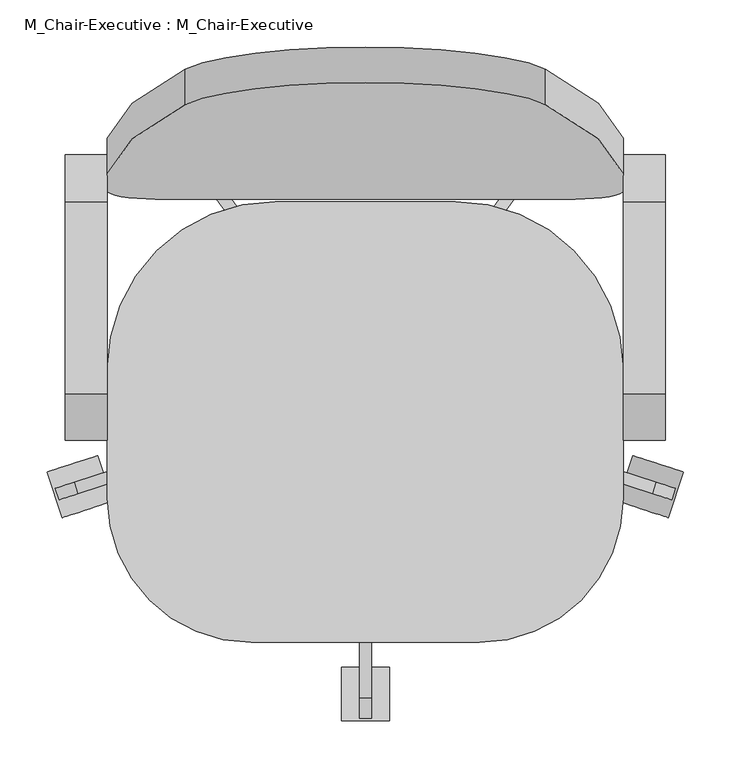
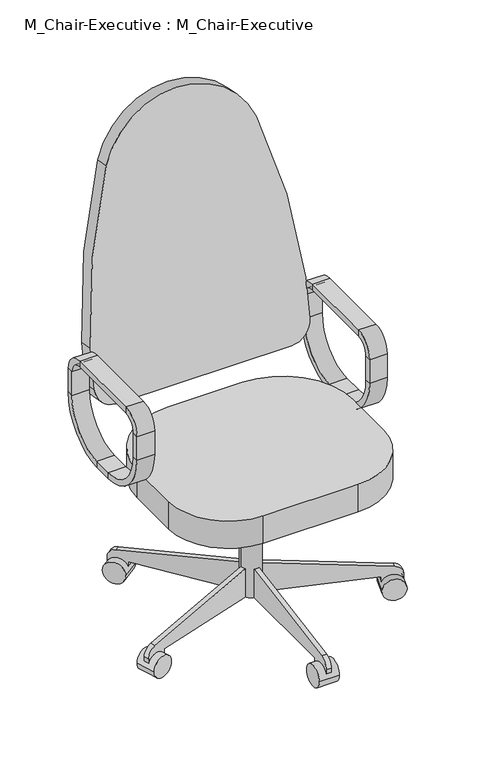
"""IFC4 building model written with IfcOpenShell, lengths in millimetres: furniture geometry, M_Chair-Executive : M_Chair-Executive."""

import ifcopenshell
import ifcopenshell.guid

model = None  # the IFC model being written
_history = None  # IfcOwnerHistory: only IFC2X3 demands one
_inside = {}  # id of a spatial element -> (the spatial element, [elements in it])
_under = {}  # id of a project, library or spatial element -> (it, [spatial elements below it])
_declared = {}  # id of a project -> (the project, [libraries it declares])
_typed = {}  # id of a type object -> (the type object, [elements of that type])
_made_of = {}  # id of a material, layer set ... -> (it, [elements and type objects made of it])


def new_model(schema):
    """Start an empty IFC model of exactly this schema.

    Asked for "IFC4X3", IfcOpenShell would pick the latest addendum, in which some entities
    have other attributes; the version numbers below select the first issue.
    IFC2X3 requires an IfcOwnerHistory on every rooted entity: one is made here for all.
    """
    global model, _history
    if schema == "IFC4X3":
        model = ifcopenshell.file(schema_version=(4, 3, 0, 0))
    else:
        model = ifcopenshell.file(schema=schema)
    _inside.clear()
    _under.clear()
    _declared.clear()
    _typed.clear()
    _made_of.clear()
    _history = None
    if model.schema == "IFC2X3":
        org = make("IfcOrganization", Name="unknown")
        user = make(
            "IfcPersonAndOrganization",
            ThePerson=make("IfcPerson", FamilyName="unknown"),
            TheOrganization=org,
        )
        app = make(
            "IfcApplication",
            ApplicationDeveloper=org,
            Version="unknown",
            ApplicationFullName="unknown",
            ApplicationIdentifier="unknown",
        )
        _history = make(
            "IfcOwnerHistory",
            OwningUser=user,
            OwningApplication=app,
            ChangeAction="ADDED",
            CreationDate=0,
        )
    return model


def make(cls, **values):
    """One entity of the class cls with the attributes given. An attribute that is None is left unset."""
    return model.create_entity(
        cls, **{name: value for name, value in values.items() if value is not None}
    )


def rooted(cls, **values):
    """An entity with a GlobalId (a new one), such as an element, a storey or a relation."""
    return make(cls, GlobalId=ifcopenshell.guid.new(), OwnerHistory=_history, **values)


def si_unit(unit_type, name, prefix=None):
    """IfcSIUnit, for example si_unit("LENGTHUNIT", "METRE", prefix="MILLI")."""
    return make("IfcSIUnit", UnitType=unit_type, Prefix=prefix, Name=name)


def assignment(units):
    """IfcUnitAssignment: the units of a project."""
    return None if units is None else make("IfcUnitAssignment", Units=units)


def point(xyz):
    """IfcCartesianPoint."""
    return None if xyz is None else make("IfcCartesianPoint", Coordinates=xyz)


def direction(xyz):
    """IfcDirection."""
    return None if xyz is None else make("IfcDirection", DirectionRatios=xyz)


def frame(location, z_axis=None, x_axis=None):
    """IfcAxis2Placement3D, a coordinate frame: its origin and axes. An axis left out is left unset."""
    return make(
        "IfcAxis2Placement3D",
        Location=point(location),
        Axis=direction(z_axis),
        RefDirection=direction(x_axis),
    )


def frame_2d(location, x_axis=None):
    """IfcAxis2Placement2D, a coordinate frame in the plane: its origin and x axis."""
    return make(
        "IfcAxis2Placement2D", Location=point(location), RefDirection=direction(x_axis)
    )


def origin():
    """The frame at (0, 0, 0) with its axes left unset."""
    return frame((0.0, 0.0, 0.0))


def place(relative_to, where):
    """IfcLocalPlacement: puts the frame where relative to a parent placement (None: the world)."""
    return make(
        "IfcLocalPlacement", PlacementRelTo=relative_to, RelativePlacement=where
    )


def context(
    kind, dimensions, precision=None, world=None, true_north=None, identifier=None
):
    """IfcGeometricRepresentationContext, for example the 3D "Model" context."""
    return make(
        "IfcGeometricRepresentationContext",
        ContextIdentifier=identifier,
        ContextType=kind,
        CoordinateSpaceDimension=dimensions,
        Precision=precision,
        WorldCoordinateSystem=world,
        TrueNorth=true_north,
    )


def project(units=None, contexts=None):
    """IfcProject with its units and contexts."""
    return rooted(
        "IfcProject",
        Name="project",
        RepresentationContexts=contexts,
        UnitsInContext=assignment(units),
    )


def spatial(cls, under=None, at=None, **own):
    """A site, building, storey or space (cls), placed at a placement, below another one or the project."""
    s = rooted(cls, ObjectPlacement=at, **own)
    if under is not None:
        _under.setdefault(under.id(), (under, []))[1].append(s)
    return s


def polyline(points):
    """IfcPolyline through the points."""
    return make("IfcPolyline", Points=[point(p) for p in points])


def circle_curve(where, radius):
    """IfcCircle in the frame where."""
    return make("IfcCircle", Position=where, Radius=radius)


def trimmed(basis, trim1, trim2, sense, master):
    """IfcTrimmedCurve: the piece of a basis curve between two trims."""
    return make(
        "IfcTrimmedCurve",
        BasisCurve=basis,
        Trim1=trim1,
        Trim2=trim2,
        SenseAgreement=sense,
        MasterRepresentation=master,
    )


def segment(curve, same_sense, transition):
    """IfcCompositeCurveSegment."""
    return make(
        "IfcCompositeCurveSegment",
        Transition=transition,
        SameSense=same_sense,
        ParentCurve=curve,
    )


def composite_curve(segments, self_intersect=None):
    """IfcCompositeCurve: segments joined end to end."""
    return make("IfcCompositeCurve", Segments=segments, SelfIntersect=self_intersect)


def outline(outer, holes=None, kind="AREA"):
    """IfcArbitraryClosedProfileDef: a profile drawn as a closed curve; with holes, ...WithVoids."""
    if holes is None:
        return make("IfcArbitraryClosedProfileDef", ProfileType=kind, OuterCurve=outer)
    return make(
        "IfcArbitraryProfileDefWithVoids",
        ProfileType=kind,
        OuterCurve=outer,
        InnerCurves=holes,
    )


def extrude(swept, where, along, depth):
    """IfcExtrudedAreaSolid: the profile swept, set in the frame where, extruded along a direction by depth."""
    return make(
        "IfcExtrudedAreaSolid",
        SweptArea=swept,
        Position=where,
        ExtrudedDirection=direction(along),
        Depth=depth,
    )


def shape(context_of_items, identifier, shape_type, items):
    """IfcShapeRepresentation: the items that make up one representation, for example the "Body"."""
    return make(
        "IfcShapeRepresentation",
        ContextOfItems=context_of_items,
        RepresentationIdentifier=identifier,
        RepresentationType=shape_type,
        Items=items,
    )


def source(mapping_origin, context_of_items, identifier, shape_type, items):
    """IfcRepresentationMap: a shape defined once, which mapped items show again and again."""
    return make(
        "IfcRepresentationMap",
        MappingOrigin=mapping_origin,
        MappedRepresentation=shape(context_of_items, identifier, shape_type, items),
    )


def transform(
    local_origin,
    x_axis=None,
    y_axis=None,
    z_axis=None,
    scale=None,
    scale2=None,
    scale3=None,
    uniform=True,
):
    """IfcCartesianTransformationOperator3D, or its non-uniform kind. x_axis, y_axis, z_axis: its Axis1, 2, 3."""
    if uniform:
        return make(
            "IfcCartesianTransformationOperator3D",
            Axis1=direction(x_axis),
            Axis2=direction(y_axis),
            LocalOrigin=point(local_origin),
            Scale=scale,
            Axis3=direction(z_axis),
        )
    return make(
        "IfcCartesianTransformationOperator3DnonUniform",
        Axis1=direction(x_axis),
        Axis2=direction(y_axis),
        LocalOrigin=point(local_origin),
        Scale=scale,
        Axis3=direction(z_axis),
        Scale2=scale2,
        Scale3=scale3,
    )


def mapped(mapping_source, mapping_target):
    """IfcMappedItem: shows the shape of a source again, moved by a transform."""
    return make(
        "IfcMappedItem", MappingSource=mapping_source, MappingTarget=mapping_target
    )


def made_of(thing, what):
    """Note that an element or type object is made of a material, layer set ...; save() writes the relation."""
    if what is not None:
        _made_of.setdefault(what.id(), (what, []))[1].append(thing)
    return thing


def element(
    cls,
    number,
    at=None,
    inside=None,
    cuts=None,
    type_object=None,
    material=None,
    context=None,
    identifier="Body",
    shape_type=None,
    held_by="IfcProductDefinitionShape",
    body=None,
    shapes=None,
    **own,
):
    """One element of the class cls, such as IfcWall. Its Tag is "e" and its number.

    at: its placement. inside: the storey or other place that contains it. cuts: it is an
    opening in that element (IfcRelVoidsElement). A single representation is given by context,
    identifier, shape_type and body (its items); several are given by shapes. held_by: the class
    of the entity that holds the representations. save() writes the other relations.
    """
    e = rooted(cls, Tag="e%d" % number, ObjectPlacement=at, **own)
    if body is not None:
        shapes = [shape(context, identifier, shape_type, body)]
    if shapes is not None:
        e.Representation = make(held_by, Representations=shapes)
    if inside is not None:
        _inside.setdefault(inside.id(), (inside, []))[1].append(e)
    if cuts is not None:
        rooted(
            "IfcRelVoidsElement", RelatingBuildingElement=cuts, RelatedOpeningElement=e
        )
    if type_object is not None:
        _typed.setdefault(type_object.id(), (type_object, []))[1].append(e)
    return made_of(e, material)


def aggregate(whole, parts):
    """IfcRelAggregates: a whole, such as a stair, and the parts it consists of."""
    return rooted("IfcRelAggregates", RelatingObject=whole, RelatedObjects=parts)


def save(model, path):
    """Write the relations noted so far, then the file.

    IfcRelAggregates (storeys below a building ...), IfcRelContainedInSpatialStructure (elements
    in a storey), IfcRelDefinesByType, IfcRelAssociatesMaterial and IfcRelDeclares: one each for
    every whole, place, type object, material and project.
    """
    for whole, parts in _under.values():
        aggregate(whole, parts)
    for where, things in _inside.values():
        rooted(
            "IfcRelContainedInSpatialStructure",
            RelatedElements=things,
            RelatingStructure=where,
        )
    for kind, things in _typed.values():
        rooted("IfcRelDefinesByType", RelatedObjects=things, RelatingType=kind)
    for what, things in _made_of.values():
        rooted("IfcRelAssociatesMaterial", RelatedObjects=things, RelatingMaterial=what)
    for by, libraries in _declared.values():
        rooted("IfcRelDeclares", RelatingContext=by, RelatedDefinitions=libraries)
    model.write(path)


def plane_surface(at):
    """IfcPlane: the flat surface through the origin of the frame at, square to its z axis."""
    return make("IfcPlane", Position=at)


def cylinder_surface(at, radius):
    """IfcCylindricalSurface: all points at the distance radius from the z axis of the frame at."""
    return make("IfcCylindricalSurface", Position=at, Radius=radius)


def revolved_surface(curve, axis_point, axis_direction):
    """IfcSurfaceOfRevolution: the curve turned about the line through axis_point along axis_direction."""
    return make(
        "IfcSurfaceOfRevolution",
        SweptCurve=make("IfcArbitraryOpenProfileDef", ProfileType="CURVE", Curve=curve),
        AxisPosition=make("IfcAxis1Placement", Location=point(axis_point), Axis=direction(axis_direction)),
    )


def advanced_brep(points, edges, surfaces, faces):
    """IfcAdvancedBrep: a solid bounded by faces that lie on surfaces and meet in shared edges.

    An edge is (start, end): straight between two places in points (the first is 0);
    or (start, end, curve); or (start, end, curve, False) where it runs against its curve.
    A face is (place in surfaces, loops), or (place, loops, False) where it looks against
    its surface's normal. A loop lists edges by number (the first is 1), with a minus sign
    where the edge is run from its end to its start. The first loop is the outer one.
    """
    corners = [point(p) for p in points]
    vertices = [make("IfcVertexPoint", VertexGeometry=c) for c in corners]
    made = []
    for start, end, *more in edges:
        made.append(
            make(
                "IfcEdgeCurve",
                EdgeStart=vertices[start],
                EdgeEnd=vertices[end],
                EdgeGeometry=more[0] if more else make("IfcPolyline", Points=[corners[start], corners[end]]),
                SameSense=more[1] if len(more) > 1 else True,
            )
        )
    hull = []
    for where, loops, *sense in faces:
        bounds = []
        for j, loop in enumerate(loops):
            ring = [make("IfcOrientedEdge", EdgeElement=made[abs(k) - 1], Orientation=k > 0) for k in loop]
            bounds.append(
                make(
                    "IfcFaceOuterBound" if j == 0 else "IfcFaceBound",
                    Bound=make("IfcEdgeLoop", EdgeList=ring),
                    Orientation=True,
                )
            )
        hull.append(make("IfcAdvancedFace", Bounds=bounds, FaceSurface=surfaces[where], SameSense=sense[0] if sense else True))
    return make("IfcAdvancedBrep", Outer=make("IfcClosedShell", CfsFaces=hull))


def m_chair_executive_m_chair_executive_a5be4872(model_context):
    return source(origin(), model_context, "Body", "SolidModel", [
        advanced_brep(
        [(-176.5091803, 217.7873012, 546.1), (-176.5091803, 233.6623012, 546.1), (-176.5091803, 108.0540984, 420.4917972), (-176.5091803, 108.0540984, 436.3667972), (-132.0591803, 217.7873012, 546.1), (-132.0591803, 108.0540984, 436.3667972), (-132.0591803, 233.6623012, 546.1), (-132.0591803, 108.0540984, 420.4917972), (-176.5091803, 217.7873012, 609.6), (-176.5091803, 233.6623012, 609.6), (-132.0591803, 217.7873012, 609.6), (-132.0591803, 233.6623012, 609.6), (-176.5091803, 184.2540984, 643.1332028), (-176.5091803, 184.2540984, 659.0082028), (-132.0591803, 184.2540984, 643.1332028), (-132.0591803, 184.2540984, 659.0082028), (-176.5091803, -18.9459016, 643.1332028), (-176.5091803, -18.9459016, 659.0082028), (-132.0591803, -18.9459016, 643.1332028), (-132.0591803, -18.9459016, 659.0082028), (-176.5091803, -52.4791044, 609.6), (-176.5091803, -68.3541044, 609.6), (-132.0591803, -52.4791044, 609.6), (-132.0591803, -68.3541044, 609.6), (-176.5091803, -52.4791044, 546.1), (-176.5091803, -68.3541044, 546.1), (-132.0591803, -52.4791044, 546.1), (-132.0591803, -68.3541044, 546.1), (-176.5091803, 57.2540984, 436.3667972), (-176.5091803, 57.2540984, 420.4917972), (-132.0591803, 57.2540984, 436.3667972), (-132.0591803, 57.2540984, 420.4917972)],
        [
            (0, 1),
            (1, 2, circle_curve(frame((-176.5091803, 108.0540984, 546.1), z_axis=(-1.0, 0.0, 0.0), x_axis=(0.0, 0.0, -1.0)), 125.6082028)),
            (2, 3),
            (3, 0, circle_curve(frame((-176.5091803, 108.0540984, 546.1), z_axis=(1.0, 0.0, 0.0), x_axis=(0.0, 0.0, -1.0)), 109.7332028)),
            (4, 0),
            (3, 5),
            (5, 4, circle_curve(frame((-132.0591803, 108.0540984, 546.1), z_axis=(1.0, 0.0, 0.0), x_axis=(0.0, 0.0, -1.0)), 109.7332028)),
            (6, 4),
            (5, 7),
            (7, 6, circle_curve(frame((-132.0591803, 108.0540984, 546.1), z_axis=(1.0, 0.0, 0.0), x_axis=(0.0, 0.0, -1.0)), 125.6082028)),
            (1, 6),
            (7, 2),
            (0, 8),
            (8, 9),
            (9, 1),
            (4, 10),
            (10, 8),
            (6, 11),
            (11, 10),
            (9, 11),
            (12, 13),
            (13, 9, circle_curve(frame((-176.5091803, 184.2540984, 609.6), z_axis=(-1.0, 0.0, 0.0), x_axis=(0.0, 1.0, 0.0)), 49.4082028)),
            (8, 12, circle_curve(frame((-176.5091803, 184.2540984, 609.6), z_axis=(1.0, 0.0, 0.0), x_axis=(0.0, 1.0, 0.0)), 33.5332028)),
            (14, 12),
            (10, 14, circle_curve(frame((-132.0591803, 184.2540984, 609.6), z_axis=(1.0, 0.0, 0.0), x_axis=(0.0, 1.0, 0.0)), 33.5332028)),
            (15, 14),
            (11, 15, circle_curve(frame((-132.0591803, 184.2540984, 609.6), z_axis=(1.0, 0.0, 0.0), x_axis=(0.0, 1.0, 0.0)), 49.4082028)),
            (13, 15),
            (12, 16),
            (16, 17),
            (17, 13),
            (14, 18),
            (18, 16),
            (15, 19),
            (19, 18),
            (17, 19),
            (20, 21),
            (21, 17, circle_curve(frame((-176.5091803, -18.9459016, 609.6), z_axis=(-1.0, 0.0, 0.0), x_axis=(0.0, 0.0, 1.0)), 49.4082028)),
            (16, 20, circle_curve(frame((-176.5091803, -18.9459016, 609.6), z_axis=(1.0, 0.0, 0.0), x_axis=(0.0, 0.0, 1.0)), 33.5332028)),
            (22, 20),
            (18, 22, circle_curve(frame((-132.0591803, -18.9459016, 609.6), z_axis=(1.0, 0.0, 0.0), x_axis=(0.0, 0.0, 1.0)), 33.5332028)),
            (23, 22),
            (19, 23, circle_curve(frame((-132.0591803, -18.9459016, 609.6), z_axis=(1.0, 0.0, 0.0), x_axis=(0.0, 0.0, 1.0)), 49.4082028)),
            (21, 23),
            (20, 24),
            (24, 25),
            (25, 21),
            (22, 26),
            (26, 24),
            (23, 27),
            (27, 26),
            (25, 27),
            (28, 29),
            (29, 25, circle_curve(frame((-176.5091803, 57.2540984, 546.1), z_axis=(-1.0, 0.0, 0.0), x_axis=(0.0, -1.0, 0.0)), 125.6082028)),
            (24, 28, circle_curve(frame((-176.5091803, 57.2540984, 546.1), z_axis=(1.0, 0.0, 0.0), x_axis=(0.0, -1.0, 0.0)), 109.7332028)),
            (30, 28),
            (26, 30, circle_curve(frame((-132.0591803, 57.2540984, 546.1), z_axis=(1.0, 0.0, 0.0), x_axis=(0.0, -1.0, 0.0)), 109.7332028)),
            (31, 30),
            (27, 31, circle_curve(frame((-132.0591803, 57.2540984, 546.1), z_axis=(1.0, 0.0, 0.0), x_axis=(0.0, -1.0, 0.0)), 125.6082028)),
            (29, 31),
            (28, 3),
            (2, 29),
            (30, 5),
            (31, 7),
        ],
        [
            plane_surface(frame((-176.5091803, 108.0540984, 546.1), z_axis=(-1.0, 0.0, 0.0), x_axis=(0.0, 0.0, -1.0))),
            revolved_surface(polyline([(-176.5091803, 108.0540984, 436.3667972), (-132.0591803, 108.0540984, 436.3667972)]), (-132.0591803, 108.0540984, 546.1), (-1.0, 0.0, 0.0)),
            plane_surface(frame((-132.0591803, 108.0540984, 546.1), z_axis=(1.0, 0.0, 0.0), x_axis=(0.0, 0.0, -1.0))),
            cylinder_surface(frame((-132.0591803, 108.0540984, 546.1), z_axis=(-1.0, 0.0, 0.0), x_axis=(0.0, 0.0, -1.0)), 125.6082028),
            plane_surface(frame((-176.5091803, 233.6623012, 546.1), z_axis=(-1.0, 0.0, 0.0), x_axis=(0.0, 0.0, 1.0))),
            plane_surface(frame((-176.5091803, 217.7873012, 546.1), z_axis=(0.0, -1.0, 0.0), x_axis=(0.0, 0.0, 1.0))),
            plane_surface(frame((-132.0591803, 217.7873012, 546.1), z_axis=(1.0, 0.0, 0.0), x_axis=(0.0, 0.0, 1.0))),
            plane_surface(frame((-132.0591803, 233.6623012, 546.1), z_axis=(0.0, 1.0, 0.0), x_axis=(0.0, 0.0, 1.0))),
            plane_surface(frame((-176.5091803, 184.2540984, 609.6), z_axis=(-1.0, 0.0, 0.0), x_axis=(0.0, 1.0, 0.0))),
            revolved_surface(polyline([(-176.5091803, 217.7873012, 609.6), (-132.0591803, 217.7873012, 609.6)]), (-132.0591803, 184.2540984, 609.6), (-1.0, 0.0, 0.0)),
            plane_surface(frame((-132.0591803, 184.2540984, 609.6), z_axis=(1.0, 0.0, 0.0), x_axis=(0.0, 1.0, 0.0))),
            cylinder_surface(frame((-132.0591803, 184.2540984, 609.6), z_axis=(-1.0, 0.0, 0.0), x_axis=(0.0, 1.0, 0.0)), 49.4082028),
            plane_surface(frame((-176.5091803, 184.2540984, 659.0082028), z_axis=(-1.0, 0.0, 0.0), x_axis=(0.0, -1.0, 0.0))),
            plane_surface(frame((-176.5091803, 184.2540984, 643.1332028), z_axis=(0.0, 0.0, -1.0), x_axis=(0.0, -1.0, 0.0))),
            plane_surface(frame((-132.0591803, 184.2540984, 643.1332028), z_axis=(1.0, 0.0, 0.0), x_axis=(0.0, -1.0, 0.0))),
            plane_surface(frame((-132.0591803, 184.2540984, 659.0082028), z_axis=(0.0, 0.0, 1.0), x_axis=(0.0, -1.0, 0.0))),
            plane_surface(frame((-176.5091803, -18.9459016, 609.6), z_axis=(-1.0, 0.0, 0.0), x_axis=(0.0, 0.0, 1.0))),
            revolved_surface(polyline([(-176.5091803, -18.9459016, 643.1332028), (-132.0591803, -18.9459016, 643.1332028)]), (-132.0591803, -18.9459016, 609.6), (-1.0, 0.0, 0.0)),
            plane_surface(frame((-132.0591803, -18.9459016, 609.6), z_axis=(1.0, 0.0, 0.0), x_axis=(0.0, 0.0, 1.0))),
            cylinder_surface(frame((-132.0591803, -18.9459016, 609.6), z_axis=(-1.0, 0.0, 0.0), x_axis=(0.0, 0.0, 1.0)), 49.4082028),
            plane_surface(frame((-176.5091803, -68.3541044, 609.6), z_axis=(-1.0, 0.0, 0.0), x_axis=(0.0, 0.0, -1.0))),
            plane_surface(frame((-176.5091803, -52.4791044, 609.6), z_axis=(0.0, 1.0, 0.0), x_axis=(0.0, 0.0, -1.0))),
            plane_surface(frame((-132.0591803, -52.4791044, 609.6), z_axis=(1.0, 0.0, 0.0), x_axis=(0.0, 0.0, -1.0))),
            plane_surface(frame((-132.0591803, -68.3541044, 609.6), z_axis=(0.0, -1.0, 0.0), x_axis=(0.0, 0.0, -1.0))),
            plane_surface(frame((-176.5091803, 57.2540984, 546.1), z_axis=(-1.0, 0.0, 0.0), x_axis=(0.0, -1.0, 0.0))),
            revolved_surface(polyline([(-176.5091803, -52.479104400000004, 546.1), (-132.0591803, -52.479104400000004, 546.1)]), (-132.0591803, 57.2540984, 546.1), (-1.0, 0.0, 0.0)),
            plane_surface(frame((-132.0591803, 57.2540984, 546.1), z_axis=(1.0, 0.0, 0.0), x_axis=(0.0, -1.0, 0.0))),
            cylinder_surface(frame((-132.0591803, 57.2540984, 546.1), z_axis=(-1.0, 0.0, 0.0), x_axis=(0.0, -1.0, 0.0)), 125.6082028),
            plane_surface(frame((-176.5091803, 57.2540984, 420.4917972), z_axis=(-1.0, 0.0, 0.0), x_axis=(0.0, 1.0, 0.0))),
            plane_surface(frame((-176.5091803, 57.2540984, 436.3667972), z_axis=(0.0, 0.0, 1.0), x_axis=(0.0, 1.0, 0.0))),
            plane_surface(frame((-132.0591803, 57.2540984, 436.3667972), z_axis=(1.0, 0.0, 0.0), x_axis=(0.0, 1.0, 0.0))),
            plane_surface(frame((-132.0591803, 57.2540984, 420.4917972), z_axis=(0.0, 0.0, -1.0), x_axis=(0.0, 1.0, 0.0))),
        ],
        [
            (0, [[1, 2, 3, 4]]),
            (1, [[5, -4, 6, 7]]),
            (2, [[8, -7, 9, 10]]),
            (3, [[11, -10, 12, -2]]),
            (4, [[13, 14, 15, -1]]),
            (5, [[16, 17, -13, -5]]),
            (6, [[18, 19, -16, -8]]),
            (7, [[-15, 20, -18, -11]]),
            (8, [[21, 22, -14, 23]]),
            (9, [[24, -23, -17, 25]]),
            (10, [[26, -25, -19, 27]]),
            (11, [[28, -27, -20, -22]]),
            (12, [[29, 30, 31, -21]]),
            (13, [[32, 33, -29, -24]]),
            (14, [[34, 35, -32, -26]]),
            (15, [[-31, 36, -34, -28]]),
            (16, [[37, 38, -30, 39]]),
            (17, [[40, -39, -33, 41]]),
            (18, [[42, -41, -35, 43]]),
            (19, [[44, -43, -36, -38]]),
            (20, [[45, 46, 47, -37]]),
            (21, [[48, 49, -45, -40]]),
            (22, [[50, 51, -48, -42]]),
            (23, [[-47, 52, -50, -44]]),
            (24, [[53, 54, -46, 55]]),
            (25, [[56, -55, -49, 57]]),
            (26, [[58, -57, -51, 59]]),
            (27, [[60, -59, -52, -54]]),
            (28, [[61, -3, 62, -53]]),
            (29, [[63, -6, -61, -56]]),
            (30, [[64, -9, -63, -58]]),
            (31, [[-62, -12, -64, -60]]),
        ],
    ),
        advanced_brep(
        [(414.0408197, 233.6623012, 546.1), (458.4908197, 233.6623012, 546.1), (458.4908197, 108.0540984, 420.4917972), (414.0408197, 108.0540984, 420.4917972), (414.0408197, 217.7873012, 546.1), (414.0408197, 108.0540984, 436.3667972), (458.4908197, 217.7873012, 546.1), (458.4908197, 108.0540984, 436.3667972), (414.0408197, 233.6623012, 609.6), (458.4908197, 233.6623012, 609.6), (414.0408197, 217.7873012, 609.6), (458.4908197, 217.7873012, 609.6), (414.0408197, 184.2540984, 659.0082028), (458.4908197, 184.2540984, 659.0082028), (414.0408197, 184.2540984, 643.1332028), (458.4908197, 184.2540984, 643.1332028), (414.0408197, -18.9459016, 659.0082028), (458.4908197, -18.9459016, 659.0082028), (414.0408197, -18.9459016, 643.1332028), (458.4908197, -18.9459016, 643.1332028), (414.0408197, -68.3541044, 609.6), (458.4908197, -68.3541044, 609.6), (414.0408197, -52.4791044, 609.6), (458.4908197, -52.4791044, 609.6), (414.0408197, -68.3541044, 546.1), (458.4908197, -68.3541044, 546.1), (414.0408197, -52.4791044, 546.1), (458.4908197, -52.4791044, 546.1), (414.0408197, 57.2540984, 420.4917972), (458.4908197, 57.2540984, 420.4917972), (414.0408197, 57.2540984, 436.3667972), (458.4908197, 57.2540984, 436.3667972)],
        [
            (0, 1),
            (1, 2, circle_curve(frame((458.4908197, 108.0540984, 546.1), z_axis=(-1.0, 0.0, 0.0), x_axis=(0.0, 0.0, -1.0)), 125.6082028)),
            (2, 3),
            (3, 0, circle_curve(frame((414.0408197, 108.0540984, 546.1), z_axis=(1.0, 0.0, 0.0), x_axis=(0.0, 0.0, -1.0)), 125.6082028)),
            (4, 0),
            (3, 5),
            (5, 4, circle_curve(frame((414.0408197, 108.0540984, 546.1), z_axis=(1.0, 0.0, 0.0), x_axis=(0.0, 0.0, -1.0)), 109.7332028)),
            (6, 4),
            (5, 7),
            (7, 6, circle_curve(frame((458.4908197, 108.0540984, 546.1), z_axis=(1.0, 0.0, 0.0), x_axis=(0.0, 0.0, -1.0)), 109.7332028)),
            (1, 6),
            (7, 2),
            (0, 8),
            (8, 9),
            (9, 1),
            (4, 10),
            (10, 8),
            (6, 11),
            (11, 10),
            (9, 11),
            (12, 13),
            (13, 9, circle_curve(frame((458.4908197, 184.2540984, 609.6), z_axis=(-1.0, 0.0, 0.0), x_axis=(0.0, 1.0, 0.0)), 49.4082028)),
            (8, 12, circle_curve(frame((414.0408197, 184.2540984, 609.6), z_axis=(1.0, 0.0, 0.0), x_axis=(0.0, 1.0, 0.0)), 49.4082028)),
            (14, 12),
            (10, 14, circle_curve(frame((414.0408197, 184.2540984, 609.6), z_axis=(1.0, 0.0, 0.0), x_axis=(0.0, 1.0, 0.0)), 33.5332028)),
            (15, 14),
            (11, 15, circle_curve(frame((458.4908197, 184.2540984, 609.6), z_axis=(1.0, 0.0, 0.0), x_axis=(0.0, 1.0, 0.0)), 33.5332028)),
            (13, 15),
            (12, 16),
            (16, 17),
            (17, 13),
            (14, 18),
            (18, 16),
            (15, 19),
            (19, 18),
            (17, 19),
            (20, 21),
            (21, 17, circle_curve(frame((458.4908197, -18.9459016, 609.6), z_axis=(-1.0, 0.0, 0.0), x_axis=(0.0, 0.0, 1.0)), 49.4082028)),
            (16, 20, circle_curve(frame((414.0408197, -18.9459016, 609.6), z_axis=(1.0, 0.0, 0.0), x_axis=(0.0, 0.0, 1.0)), 49.4082028)),
            (22, 20),
            (18, 22, circle_curve(frame((414.0408197, -18.9459016, 609.6), z_axis=(1.0, 0.0, 0.0), x_axis=(0.0, 0.0, 1.0)), 33.5332028)),
            (23, 22),
            (19, 23, circle_curve(frame((458.4908197, -18.9459016, 609.6), z_axis=(1.0, 0.0, 0.0), x_axis=(0.0, 0.0, 1.0)), 33.5332028)),
            (21, 23),
            (20, 24),
            (24, 25),
            (25, 21),
            (22, 26),
            (26, 24),
            (23, 27),
            (27, 26),
            (25, 27),
            (28, 29),
            (29, 25, circle_curve(frame((458.4908197, 57.2540984, 546.1), z_axis=(-1.0, 0.0, 0.0), x_axis=(0.0, -1.0, 0.0)), 125.6082028)),
            (24, 28, circle_curve(frame((414.0408197, 57.2540984, 546.1), z_axis=(1.0, 0.0, 0.0), x_axis=(0.0, -1.0, 0.0)), 125.6082028)),
            (30, 28),
            (26, 30, circle_curve(frame((414.0408197, 57.2540984, 546.1), z_axis=(1.0, 0.0, 0.0), x_axis=(0.0, -1.0, 0.0)), 109.7332028)),
            (31, 30),
            (27, 31, circle_curve(frame((458.4908197, 57.2540984, 546.1), z_axis=(1.0, 0.0, 0.0), x_axis=(0.0, -1.0, 0.0)), 109.7332028)),
            (29, 31),
            (28, 3),
            (2, 29),
            (30, 5),
            (31, 7),
        ],
        [
            cylinder_surface(frame((414.0408197, 108.0540984, 546.1), z_axis=(-1.0, 0.0, 0.0), x_axis=(0.0, 0.0, -1.0)), 125.6082028),
            plane_surface(frame((414.0408197, 108.0540984, 546.1), z_axis=(-1.0, 0.0, 0.0), x_axis=(0.0, 0.0, -1.0))),
            revolved_surface(polyline([(414.0408197, 108.0540984, 436.3667972), (458.4908197, 108.0540984, 436.3667972)]), (414.0408197, 108.0540984, 546.1), (-1.0, 0.0, 0.0)),
            plane_surface(frame((458.4908197, 108.0540984, 546.1), z_axis=(1.0, 0.0, 0.0), x_axis=(0.0, 0.0, -1.0))),
            plane_surface(frame((458.4908197, 233.6623012, 546.1), z_axis=(0.0, 1.0, 0.0), x_axis=(0.0, 0.0, 1.0))),
            plane_surface(frame((414.0408197, 233.6623012, 546.1), z_axis=(-1.0, 0.0, 0.0), x_axis=(0.0, 0.0, 1.0))),
            plane_surface(frame((414.0408197, 217.7873012, 546.1), z_axis=(0.0, -1.0, 0.0), x_axis=(0.0, 0.0, 1.0))),
            plane_surface(frame((458.4908197, 217.7873012, 546.1), z_axis=(1.0, 0.0, 0.0), x_axis=(0.0, 0.0, 1.0))),
            cylinder_surface(frame((414.0408197, 184.2540984, 609.6), z_axis=(-1.0, 0.0, 0.0), x_axis=(0.0, 1.0, 0.0)), 49.4082028),
            plane_surface(frame((414.0408197, 184.2540984, 609.6), z_axis=(-1.0, 0.0, 0.0), x_axis=(0.0, 1.0, 0.0))),
            revolved_surface(polyline([(414.0408197, 217.7873012, 609.6), (458.4908197, 217.7873012, 609.6)]), (414.0408197, 184.2540984, 609.6), (-1.0, 0.0, 0.0)),
            plane_surface(frame((458.4908197, 184.2540984, 609.6), z_axis=(1.0, 0.0, 0.0), x_axis=(0.0, 1.0, 0.0))),
            plane_surface(frame((458.4908197, 184.2540984, 659.0082028), z_axis=(0.0, 0.0, 1.0), x_axis=(0.0, -1.0, 0.0))),
            plane_surface(frame((414.0408197, 184.2540984, 659.0082028), z_axis=(-1.0, 0.0, 0.0), x_axis=(0.0, -1.0, 0.0))),
            plane_surface(frame((414.0408197, 184.2540984, 643.1332028), z_axis=(0.0, 0.0, -1.0), x_axis=(0.0, -1.0, 0.0))),
            plane_surface(frame((458.4908197, 184.2540984, 643.1332028), z_axis=(1.0, 0.0, 0.0), x_axis=(0.0, -1.0, 0.0))),
            cylinder_surface(frame((414.0408197, -18.9459016, 609.6), z_axis=(-1.0, 0.0, 0.0), x_axis=(0.0, 0.0, 1.0)), 49.4082028),
            plane_surface(frame((414.0408197, -18.9459016, 609.6), z_axis=(-1.0, 0.0, 0.0), x_axis=(0.0, 0.0, 1.0))),
            revolved_surface(polyline([(414.0408197, -18.9459016, 643.1332028), (458.4908197, -18.9459016, 643.1332028)]), (414.0408197, -18.9459016, 609.6), (-1.0, 0.0, 0.0)),
            plane_surface(frame((458.4908197, -18.9459016, 609.6), z_axis=(1.0, 0.0, 0.0), x_axis=(0.0, 0.0, 1.0))),
            plane_surface(frame((458.4908197, -68.3541044, 609.6), z_axis=(0.0, -1.0, 0.0), x_axis=(0.0, 0.0, -1.0))),
            plane_surface(frame((414.0408197, -68.3541044, 609.6), z_axis=(-1.0, 0.0, 0.0), x_axis=(0.0, 0.0, -1.0))),
            plane_surface(frame((414.0408197, -52.4791044, 609.6), z_axis=(0.0, 1.0, 0.0), x_axis=(0.0, 0.0, -1.0))),
            plane_surface(frame((458.4908197, -52.4791044, 609.6), z_axis=(1.0, 0.0, 0.0), x_axis=(0.0, 0.0, -1.0))),
            cylinder_surface(frame((414.0408197, 57.2540984, 546.1), z_axis=(-1.0, 0.0, 0.0), x_axis=(0.0, -1.0, 0.0)), 125.6082028),
            plane_surface(frame((414.0408197, 57.2540984, 546.1), z_axis=(-1.0, 0.0, 0.0), x_axis=(0.0, -1.0, 0.0))),
            revolved_surface(polyline([(414.0408197, -52.479104400000004, 546.1), (458.4908197, -52.479104400000004, 546.1)]), (414.0408197, 57.2540984, 546.1), (-1.0, 0.0, 0.0)),
            plane_surface(frame((458.4908197, 57.2540984, 546.1), z_axis=(1.0, 0.0, 0.0), x_axis=(0.0, -1.0, 0.0))),
            plane_surface(frame((458.4908197, 57.2540984, 420.4917972), z_axis=(0.0, 0.0, -1.0), x_axis=(0.0, 1.0, 0.0))),
            plane_surface(frame((414.0408197, 57.2540984, 420.4917972), z_axis=(-1.0, 0.0, 0.0), x_axis=(0.0, 1.0, 0.0))),
            plane_surface(frame((414.0408197, 57.2540984, 436.3667972), z_axis=(0.0, 0.0, 1.0), x_axis=(0.0, 1.0, 0.0))),
            plane_surface(frame((458.4908197, 57.2540984, 436.3667972), z_axis=(1.0, 0.0, 0.0), x_axis=(0.0, 1.0, 0.0))),
        ],
        [
            (0, [[1, 2, 3, 4]]),
            (1, [[5, -4, 6, 7]]),
            (2, [[8, -7, 9, 10]]),
            (3, [[11, -10, 12, -2]]),
            (4, [[13, 14, 15, -1]]),
            (5, [[16, 17, -13, -5]]),
            (6, [[18, 19, -16, -8]]),
            (7, [[-15, 20, -18, -11]]),
            (8, [[21, 22, -14, 23]]),
            (9, [[24, -23, -17, 25]]),
            (10, [[26, -25, -19, 27]]),
            (11, [[28, -27, -20, -22]]),
            (12, [[29, 30, 31, -21]]),
            (13, [[32, 33, -29, -24]]),
            (14, [[34, 35, -32, -26]]),
            (15, [[-31, 36, -34, -28]]),
            (16, [[37, 38, -30, 39]]),
            (17, [[40, -39, -33, 41]]),
            (18, [[42, -41, -35, 43]]),
            (19, [[44, -43, -36, -38]]),
            (20, [[45, 46, 47, -37]]),
            (21, [[48, 49, -45, -40]]),
            (22, [[50, 51, -48, -42]]),
            (23, [[-47, 52, -50, -44]]),
            (24, [[53, 54, -46, 55]]),
            (25, [[56, -55, -49, 57]]),
            (26, [[58, -57, -51, 59]]),
            (27, [[60, -59, -52, -54]]),
            (28, [[61, -3, 62, -53]]),
            (29, [[63, -6, -61, -56]]),
            (30, [[64, -9, -63, -58]]),
            (31, [[-62, -12, -64, -60]]),
        ],
    ),
        extrude(outline(composite_curve([segment(polyline([(0.0, 0.0), (-444.5, 0.0)]), True, "CONTINUOUS"), segment(trimmed(circle_curve(frame_2d((-444.5, 50.8)), 50.8), [point((-444.5, 0.0))], [point((-495.3, 50.8))], False, "CARTESIAN"), True, "CONTINUOUS"), segment(polyline([(-495.3, 50.8), (-495.3, 152.4)]), True, "CONTINUOUS"), segment(trimmed(circle_curve(frame_2d((1026.7021854, 74.3913617)), 1524.0), [point((-495.3, 152.4))], [point((-412.75, 574.9444618))], False, "CARTESIAN"), True, "CONTINUOUS"), segment(trimmed(circle_curve(frame_2d((-222.25, 504.2338544)), 203.2), [point((-412.75, 574.9444618))], [point((-31.75, 574.9444618))], False, "CARTESIAN"), True, "CONTINUOUS"), segment(trimmed(circle_curve(frame_2d((-1471.2021854, 74.3913617)), 1524.0), [point((-31.75, 574.9444618))], [point((50.8, 152.4))], False, "CARTESIAN"), True, "CONTINUOUS"), segment(polyline([(50.8, 152.4), (50.8, 50.8)]), True, "CONTINUOUS"), segment(trimmed(circle_curve(frame_2d((0.0, 50.8)), 50.8), [point((50.8, 50.8))], [point((0.0, 0.0))], False, "CARTESIAN"), True, "CONTINUOUS")], self_intersect=False)), frame((363.2408197, 224.5698964, 503.1641822), z_axis=(0.0, -0.9848077530122084, 0.17364817766692853), x_axis=(1.0, 0.0, 0.0)), (0.0, 0.0, 1.0), 38.1),
        extrude(outline(composite_curve([segment(polyline([(-132.0591803, -129.4961016), (-132.0591803, 6.4540984)]), True, "CONTINUOUS"), segment(trimmed(circle_curve(frame_2d((45.7408197, 6.4540984)), 177.8), [point((-132.0591803, 6.4540984))], [point((45.7408197, 184.2540984))], False, "CARTESIAN"), True, "CONTINUOUS"), segment(polyline([(45.7408197, 184.2540984), (236.2408197, 184.2540984)]), True, "CONTINUOUS"), segment(trimmed(circle_curve(frame_2d((236.2408197, 6.4540984)), 177.8), [point((236.2408197, 184.2540984))], [point((414.0408197, 6.4540984))], False, "CARTESIAN"), True, "CONTINUOUS"), segment(polyline([(414.0408197, 6.4540984), (414.0408197, -129.4961016)]), True, "CONTINUOUS"), segment(trimmed(circle_curve(frame_2d((261.6408197, -129.4961016)), 152.4), [point((414.0408197, -129.4961016))], [point((261.6408197, -281.8961016))], False, "CARTESIAN"), True, "CONTINUOUS"), segment(polyline([(261.6408197, -281.8961016), (20.3408197, -281.8961016)]), True, "CONTINUOUS"), segment(trimmed(circle_curve(frame_2d((20.3408197, -129.4961016)), 152.4), [point((20.3408197, -281.8961016))], [point((-132.0591803, -129.4961016))], False, "CARTESIAN"), True, "CONTINUOUS")], self_intersect=False)), frame((0.0, 0.0, 383.7835944), z_axis=(0.0, 0.0, 1.0), x_axis=(1.0, 0.0, 0.0)), (0.0, 0.0, 1.0), 73.4164056),
        extrude(outline(composite_curve([segment(trimmed(circle_curve(frame_2d((140.9908197, -18.9459016)), 25.4), [point((115.5908197, -18.9459016))], [point((166.3908197, -18.9459016))], False, "CARTESIAN"), True, "CONTINUOUS"), segment(trimmed(circle_curve(frame_2d((140.9908197, -18.9459016)), 25.4), [point((166.3908197, -18.9459016))], [point((115.5908197, -18.9459016))], False, "CARTESIAN"), True, "CONTINUOUS")], self_intersect=False)), frame((0.0, 0.0, 53.5835944), z_axis=(0.0, 0.0, 1.0), x_axis=(1.0, 0.0, 0.0)), (0.0, 0.0, 1.0), 330.5914056),
        extrude(outline(composite_curve([segment(trimmed(circle_curve(frame_2d((0.0, 28.2002728)), 28.2002727), [point((0.0, 56.4005455))], [point((0.0, 0.0))], False, "CARTESIAN"), True, "CONTINUOUS"), segment(trimmed(circle_curve(frame_2d((0.0, 28.2002728)), 28.2002727), [point((0.0, 0.0))], [point((0.0, 56.4005455))], False, "CARTESIAN"), True, "CONTINUOUS")], self_intersect=False)), frame((461.9222851, -149.9299964, 28.1835944), z_axis=(0.3090169943749423, 0.9510565162951553, 0.0), x_axis=(0.0, 0.0, -1.0)), (0.0, 0.0, 1.0), 50.8),
        extrude(outline(composite_curve([segment(polyline([(25.4, 0.0), (0.0, 0.0), (0.0, 50.8), (24.303053, 50.8)]), True, "CONTINUOUS"), segment(trimmed(circle_curve(frame_2d((24.303053, 25.4)), 25.4), [point((24.303053, 50.8))], [point((49.3171699, 29.8106636))], False, "CARTESIAN"), True, "CONTINUOUS"), segment(polyline([(49.3171699, 29.8106636), (101.6, -266.7), (101.6, -292.1), (25.4, -292.1), (25.4, 0.0)]), True, "CONTINUOUS")], self_intersect=False)), frame((416.8321702, -115.2489746, 28.1835944), z_axis=(0.3090169943749423, 0.9510565162951553, 0.0), x_axis=(0.0, 0.0, 1.0)), (0.0, 0.0, 1.0), 12.7),
        extrude(outline(composite_curve([segment(trimmed(circle_curve(frame_2d((0.0, 28.2002726)), 28.2002727), [point((0.0, 56.4005454))], [point((0.0, 0.0))], False, "CARTESIAN"), True, "CONTINUOUS"), segment(trimmed(circle_curve(frame_2d((0.0, 28.2002726)), 28.2002727), [point((0.0, 0.0))], [point((0.0, 56.4005454))], False, "CARTESIAN"), True, "CONTINUOUS")], self_intersect=False)), frame((364.7373733, 245.8017485, 28.1835944), z_axis=(-0.8090169943749499, 0.5877852522924699, 0.0), x_axis=(0.0, 0.0, -1.0)), (0.0, 0.0, 1.0), 50.8),
        extrude(outline(composite_curve([segment(polyline([(25.4, 0.0), (0.0, 0.0), (0.0, 50.8), (24.303053, 50.8)]), True, "CONTINUOUS"), segment(trimmed(circle_curve(frame_2d((24.303053, 25.3999999)), 25.4), [point((24.303053, 50.8))], [point((49.3171699, 29.8106637))], False, "CARTESIAN"), True, "CONTINUOUS"), segment(polyline([(49.3171699, 29.8106637), (101.6, -266.7), (101.6, -292.1), (25.4, -292.1), (25.4, 0.0)]), True, "CONTINUOUS")], self_intersect=False)), frame((317.8201498, 213.6355261, 28.1835944), z_axis=(-0.8090169943749499, 0.5877852522924699, 0.0), x_axis=(0.0, 0.0, 1.0)), (0.0, 0.0, 1.0), 12.7),
        extrude(outline(composite_curve([segment(trimmed(circle_curve(frame_2d((0.0, 28.2002726)), 28.2002727), [point((0.0, 56.4005454))], [point((0.0, 0.0))], False, "CARTESIAN"), True, "CONTINUOUS"), segment(trimmed(circle_curve(frame_2d((0.0, 28.2002726)), 28.2002727), [point((0.0, 0.0))], [point((0.0, 56.4005454))], False, "CARTESIAN"), True, "CONTINUOUS")], self_intersect=False)), frame((-82.755734, 245.8017485, 28.1835944), z_axis=(0.8090169943749458, 0.5877852522924754, 0.0), x_axis=(0.0, 0.0, 1.0)), (0.0, 0.0, 1.0), 50.8),
        extrude(outline(composite_curve([segment(polyline([(-25.4, 0.0), (-25.4, -292.1), (-101.6, -292.1), (-101.6, -266.6999999), (-49.3171699, 29.8106637)]), True, "CONTINUOUS"), segment(trimmed(circle_curve(frame_2d((-24.303053, 25.3999999)), 25.4), [point((-49.3171699, 29.8106637))], [point((-24.303053, 50.8))], False, "CARTESIAN"), True, "CONTINUOUS"), segment(polyline([(-24.303053, 50.8), (0.0, 50.8), (0.0, 0.0), (-25.4, 0.0)]), True, "CONTINUOUS")], self_intersect=False)), frame((-35.8385104, 213.6355261, 28.1835944), z_axis=(0.8090169943749459, 0.5877852522924754, 0.0), x_axis=(0.0, 0.0, -1.0)), (0.0, 0.0, 1.0), 12.7),
        extrude(outline(composite_curve([segment(trimmed(circle_curve(frame_2d((0.0, 28.2002727)), 28.2002727), [point((0.0, 56.4005454))], [point((0.0, 0.0))], False, "CARTESIAN"), True, "CONTINUOUS"), segment(trimmed(circle_curve(frame_2d((0.0, 28.2002727)), 28.2002727), [point((0.0, 0.0))], [point((0.0, 56.4005454))], False, "CARTESIAN"), True, "CONTINUOUS")], self_intersect=False)), frame((-179.9406457, -149.9299964, 28.1835944), z_axis=(-0.3090169943749487, 0.9510565162951532, 0.0), x_axis=(0.0, 0.0, 1.0)), (0.0, 0.0, 1.0), 50.8),
        extrude(outline(composite_curve([segment(polyline([(-25.4, 0.0), (-25.4, -292.1), (-101.6, -292.1), (-101.6, -266.7), (-49.3171699, 29.8106637)]), True, "CONTINUOUS"), segment(trimmed(circle_curve(frame_2d((-24.303053, 25.4)), 25.4), [point((-49.3171699, 29.8106637))], [point((-24.303053, 50.8000001))], False, "CARTESIAN"), True, "CONTINUOUS"), segment(polyline([(-24.303053, 50.8000001), (0.0, 50.8000001), (0.0, 0.0), (-25.4, 0.0)]), True, "CONTINUOUS")], self_intersect=False)), frame((-134.8505308, -115.2489746, 28.1835944), z_axis=(-0.3090169943749487, 0.9510565162951532, 0.0), x_axis=(0.0, 0.0, -1.0)), (0.0, 0.0, 1.0), 12.7),
        extrude(outline(composite_curve([segment(trimmed(circle_curve(frame_2d((-336.4459016, 28.1835944)), 28.2002727), [point((-308.2456289, 28.1835944))], [point((-364.6461744, 28.1835944))], False, "CARTESIAN"), True, "CONTINUOUS"), segment(trimmed(circle_curve(frame_2d((-336.4459016, 28.1835944)), 28.2002727), [point((-364.6461744, 28.1835944))], [point((-308.2456289, 28.1835944))], False, "CARTESIAN"), True, "CONTINUOUS")], self_intersect=False)), frame((115.5908197, 0.0, 0.0), z_axis=(1.0, 0.0, 0.0), x_axis=(0.0, 1.0, 0.0)), (0.0, 0.0, 1.0), 50.8),
        extrude(outline(composite_curve([segment(polyline([(-311.0459016, 53.5835944), (-311.0459016, 28.1835944), (-361.8459016, 28.1835944), (-361.8459016, 52.4866474)]), True, "CONTINUOUS"), segment(trimmed(circle_curve(frame_2d((-336.4459016, 52.4866474)), 25.4), [point((-361.8459016, 52.4866474))], [point((-340.8565654, 77.5007643))], False, "CARTESIAN"), True, "CONTINUOUS"), segment(polyline([(-340.8565654, 77.5007643), (-44.3459016, 129.7835944), (-18.9459016, 129.7835944), (-18.9459016, 53.5835944), (-311.0459016, 53.5835944)]), True, "CONTINUOUS")], self_intersect=False)), frame((134.6408197, 0.0, 0.0), z_axis=(1.0, 0.0, 0.0), x_axis=(0.0, 1.0, 0.0)), (0.0, 0.0, 1.0), 12.7),
        extrude(outline(polyline([(-69.7459016, 383.7835944), (19.1540984, 383.7835944), (19.1540984, 283.0954134), (-18.9459016, 283.0954134), (-69.7459016, 371.0835944), (-69.7459016, 383.7835944)])), frame((90.1908197, 0.0, 0.0), z_axis=(1.0, 0.0, 0.0), x_axis=(0.0, 1.0, 0.0)), (0.0, 0.0, 1.0), 101.6),
    ])


if __name__ == "__main__":
    model = new_model("IFC4")
    model_context = context("Model", 3, world=origin())
    ifc_project = project(units=[si_unit("LENGTHUNIT", "METRE", prefix="MILLI")], contexts=[model_context])
    site = spatial("IfcSite", under=ifc_project)
    building = spatial("IfcBuilding", under=site)
    placement = place(None, origin())
    m_chair_executive_m_chair_executive_shape = m_chair_executive_m_chair_executive_a5be4872(model_context)
    element("IfcFurniture", 1, ObjectType="M_Chair-Executive : M_Chair-Executive", at=placement, inside=building, context=model_context, shape_type="MappedRepresentation", body=[
        mapped(m_chair_executive_m_chair_executive_shape, transform((0.0, 0.0, 0.0), x_axis=(1.0, 0.0, 0.0), y_axis=(0.0, 1.0, 0.0), z_axis=(0.0, 0.0, 1.0))),
    ])
    save(model, "model.ifc")

# Revit data of these elements
# Type "M_Chair-Executive : M_Chair-Executive"
#   Base/Armd Material = Plastic, Opaque Black
#   Caster Material = Plastic, Opaque Black
#   Seat/Back Material = Textile - Slate Blue
# Element 1 (IfcFurniture, "M_Chair-Executive : M_Chair-Executive")
#   Materials on its faces: "Plastic, Opaque Black", "Textile - Slate Blue"
# Materials
#   "Plastic, Opaque Black": class "Plastic", colour RGB 0 0 0, transparency 0.7, Description = "Plastic, generic, opaque black", Cost = 0
#   "Textile - Slate Blue": class "Fabric", colour RGB 98 102 118, transparency 0
